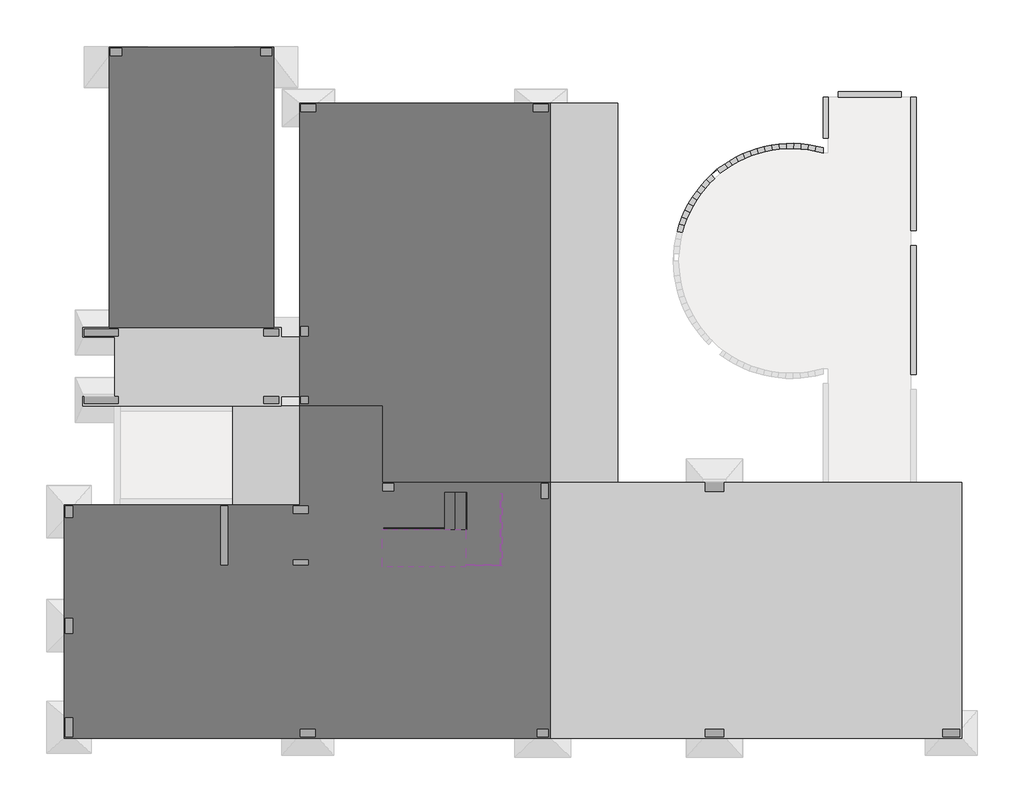
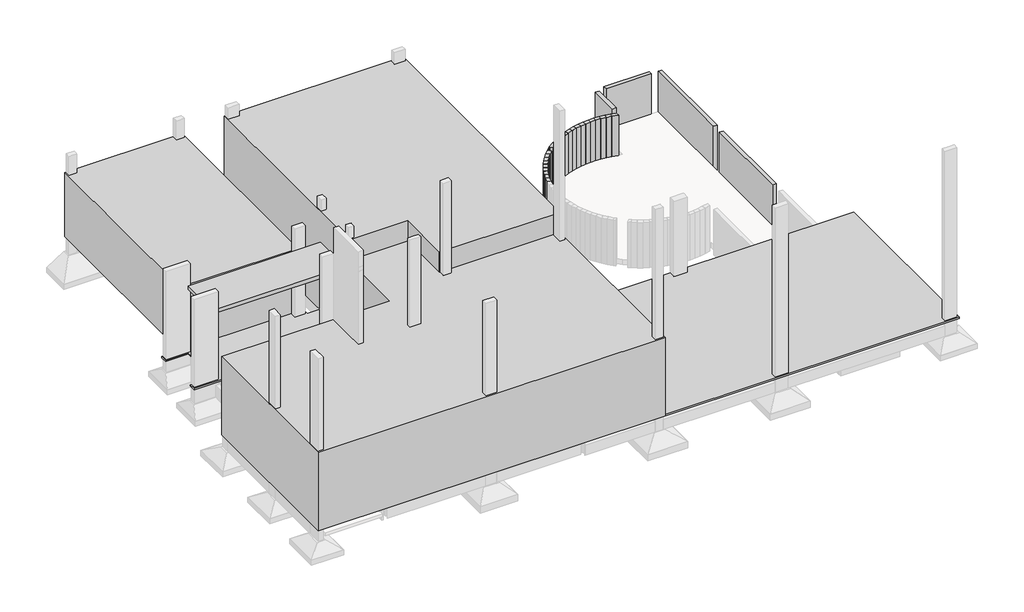
# One storey, part 4 of 4: 27 beams, 7 proxies, 6 railings, 2 stair flights, 1 slab.
"""IFC4 building model written with IfcOpenShell, lengths in millimetres."""

import ifcopenshell
import ifcopenshell.guid

model = None  # the IFC model being written
_history = None  # IfcOwnerHistory: only IFC2X3 demands one
_inside = {}  # id of a spatial element -> (the spatial element, [elements in it])
_under = {}  # id of a project, library or spatial element -> (it, [spatial elements below it])
_declared = {}  # id of a project -> (the project, [libraries it declares])
_typed = {}  # id of a type object -> (the type object, [elements of that type])
_made_of = {}  # id of a material, layer set ... -> (it, [elements and type objects made of it])


def new_model(schema):
    """Start an empty IFC model of exactly this schema.

    Asked for "IFC4X3", IfcOpenShell would pick the latest addendum, in which some entities
    have other attributes; the version numbers below select the first issue.
    IFC2X3 requires an IfcOwnerHistory on every rooted entity: one is made here for all.
    """
    global model, _history
    if schema == "IFC4X3":
        model = ifcopenshell.file(schema_version=(4, 3, 0, 0))
    else:
        model = ifcopenshell.file(schema=schema)
    _inside.clear()
    _under.clear()
    _declared.clear()
    _typed.clear()
    _made_of.clear()
    _history = None
    if model.schema == "IFC2X3":
        org = make("IfcOrganization", Name="unknown")
        user = make(
            "IfcPersonAndOrganization",
            ThePerson=make("IfcPerson", FamilyName="unknown"),
            TheOrganization=org,
        )
        app = make(
            "IfcApplication",
            ApplicationDeveloper=org,
            Version="unknown",
            ApplicationFullName="unknown",
            ApplicationIdentifier="unknown",
        )
        _history = make(
            "IfcOwnerHistory",
            OwningUser=user,
            OwningApplication=app,
            ChangeAction="ADDED",
            CreationDate=0,
        )
    return model


def make(cls, **values):
    """One entity of the class cls with the attributes given. An attribute that is None is left unset."""
    return model.create_entity(
        cls, **{name: value for name, value in values.items() if value is not None}
    )


def rooted(cls, **values):
    """An entity with a GlobalId (a new one), such as an element, a storey or a relation."""
    return make(cls, GlobalId=ifcopenshell.guid.new(), OwnerHistory=_history, **values)


def si_unit(unit_type, name, prefix=None):
    """IfcSIUnit, for example si_unit("LENGTHUNIT", "METRE", prefix="MILLI")."""
    return make("IfcSIUnit", UnitType=unit_type, Prefix=prefix, Name=name)


def assignment(units):
    """IfcUnitAssignment: the units of a project."""
    return None if units is None else make("IfcUnitAssignment", Units=units)


def point(xyz):
    """IfcCartesianPoint."""
    return None if xyz is None else make("IfcCartesianPoint", Coordinates=xyz)


def direction(xyz):
    """IfcDirection."""
    return None if xyz is None else make("IfcDirection", DirectionRatios=xyz)


def frame(location, z_axis=None, x_axis=None):
    """IfcAxis2Placement3D, a coordinate frame: its origin and axes. An axis left out is left unset."""
    return make(
        "IfcAxis2Placement3D",
        Location=point(location),
        Axis=direction(z_axis),
        RefDirection=direction(x_axis),
    )


def origin():
    """The frame at (0, 0, 0) with its axes left unset."""
    return frame((0.0, 0.0, 0.0))


def place(relative_to, where):
    """IfcLocalPlacement: puts the frame where relative to a parent placement (None: the world)."""
    return make(
        "IfcLocalPlacement", PlacementRelTo=relative_to, RelativePlacement=where
    )


def context(
    kind, dimensions, precision=None, world=None, true_north=None, identifier=None
):
    """IfcGeometricRepresentationContext, for example the 3D "Model" context."""
    return make(
        "IfcGeometricRepresentationContext",
        ContextIdentifier=identifier,
        ContextType=kind,
        CoordinateSpaceDimension=dimensions,
        Precision=precision,
        WorldCoordinateSystem=world,
        TrueNorth=true_north,
    )


def project(units=None, contexts=None):
    """IfcProject with its units and contexts."""
    return rooted(
        "IfcProject",
        Name="project",
        RepresentationContexts=contexts,
        UnitsInContext=assignment(units),
    )


def spatial(cls, under=None, at=None, **own):
    """A site, building, storey or space (cls), placed at a placement, below another one or the project."""
    s = rooted(cls, ObjectPlacement=at, **own)
    if under is not None:
        _under.setdefault(under.id(), (under, []))[1].append(s)
    return s


def polyline(points):
    """IfcPolyline through the points."""
    return make("IfcPolyline", Points=[point(p) for p in points])


def outline(outer, holes=None, kind="AREA"):
    """IfcArbitraryClosedProfileDef: a profile drawn as a closed curve; with holes, ...WithVoids."""
    if holes is None:
        return make("IfcArbitraryClosedProfileDef", ProfileType=kind, OuterCurve=outer)
    return make(
        "IfcArbitraryProfileDefWithVoids",
        ProfileType=kind,
        OuterCurve=outer,
        InnerCurves=holes,
    )


def extrude(swept, where, along, depth):
    """IfcExtrudedAreaSolid: the profile swept, set in the frame where, extruded along a direction by depth."""
    return make(
        "IfcExtrudedAreaSolid",
        SweptArea=swept,
        Position=where,
        ExtrudedDirection=direction(along),
        Depth=depth,
    )


def faces_of(points, faces, orient=None, outer=None):
    """IfcFace entities. A face is a list of loops; a loop is a list of indices into points, from 0.

    orient and outer hold one flag for each loop. By default every Orientation is true, the
    first loop of a face is its IfcFaceOuterBound and the others are IfcFaceBound.
    """
    made = []
    for i, loops in enumerate(faces):
        bounds = []
        for j, loop in enumerate(loops):
            is_outer = j == 0 if outer is None else outer[i][j]
            bounds.append(
                make(
                    "IfcFaceOuterBound" if is_outer else "IfcFaceBound",
                    Bound=make("IfcPolyLoop", Polygon=[points[k] for k in loop]),
                    Orientation=True if orient is None else orient[i][j],
                )
            )
        made.append(make("IfcFace", Bounds=bounds))
    return made


def faceted_brep(points, faces, orient=None, outer=None, voids=None):
    """IfcFacetedBrep: a solid bounded by flat faces; with voids (closed shells), ...WithVoids."""
    shared = [point(p) for p in points]
    hull = make("IfcClosedShell", CfsFaces=faces_of(shared, faces, orient, outer))
    if voids is None:
        return make("IfcFacetedBrep", Outer=hull)
    return make(
        "IfcFacetedBrepWithVoids",
        Outer=hull,
        Voids=[
            make(cls, CfsFaces=faces_of(shared, fs, o, b)) for cls, fs, o, b in voids
        ],
    )


def shape(context_of_items, identifier, shape_type, items):
    """IfcShapeRepresentation: the items that make up one representation, for example the "Body"."""
    return make(
        "IfcShapeRepresentation",
        ContextOfItems=context_of_items,
        RepresentationIdentifier=identifier,
        RepresentationType=shape_type,
        Items=items,
    )


def source(mapping_origin, context_of_items, identifier, shape_type, items):
    """IfcRepresentationMap: a shape defined once, which mapped items show again and again."""
    return make(
        "IfcRepresentationMap",
        MappingOrigin=mapping_origin,
        MappedRepresentation=shape(context_of_items, identifier, shape_type, items),
    )


def transform(
    local_origin,
    x_axis=None,
    y_axis=None,
    z_axis=None,
    scale=None,
    scale2=None,
    scale3=None,
    uniform=True,
):
    """IfcCartesianTransformationOperator3D, or its non-uniform kind. x_axis, y_axis, z_axis: its Axis1, 2, 3."""
    if uniform:
        return make(
            "IfcCartesianTransformationOperator3D",
            Axis1=direction(x_axis),
            Axis2=direction(y_axis),
            LocalOrigin=point(local_origin),
            Scale=scale,
            Axis3=direction(z_axis),
        )
    return make(
        "IfcCartesianTransformationOperator3DnonUniform",
        Axis1=direction(x_axis),
        Axis2=direction(y_axis),
        LocalOrigin=point(local_origin),
        Scale=scale,
        Axis3=direction(z_axis),
        Scale2=scale2,
        Scale3=scale3,
    )


def mapped(mapping_source, mapping_target):
    """IfcMappedItem: shows the shape of a source again, moved by a transform."""
    return make(
        "IfcMappedItem", MappingSource=mapping_source, MappingTarget=mapping_target
    )


def made_of(thing, what):
    """Note that an element or type object is made of a material, layer set ...; save() writes the relation."""
    if what is not None:
        _made_of.setdefault(what.id(), (what, []))[1].append(thing)
    return thing


def element(
    cls,
    number,
    at=None,
    inside=None,
    cuts=None,
    type_object=None,
    material=None,
    context=None,
    identifier="Body",
    shape_type=None,
    held_by="IfcProductDefinitionShape",
    body=None,
    shapes=None,
    **own,
):
    """One element of the class cls, such as IfcWall. Its Tag is "e" and its number.

    at: its placement. inside: the storey or other place that contains it. cuts: it is an
    opening in that element (IfcRelVoidsElement). A single representation is given by context,
    identifier, shape_type and body (its items); several are given by shapes. held_by: the class
    of the entity that holds the representations. save() writes the other relations.
    """
    e = rooted(cls, Tag="e%d" % number, ObjectPlacement=at, **own)
    if body is not None:
        shapes = [shape(context, identifier, shape_type, body)]
    if shapes is not None:
        e.Representation = make(held_by, Representations=shapes)
    if inside is not None:
        _inside.setdefault(inside.id(), (inside, []))[1].append(e)
    if cuts is not None:
        rooted(
            "IfcRelVoidsElement", RelatingBuildingElement=cuts, RelatedOpeningElement=e
        )
    if type_object is not None:
        _typed.setdefault(type_object.id(), (type_object, []))[1].append(e)
    return made_of(e, material)


def aggregate(whole, parts):
    """IfcRelAggregates: a whole, such as a stair, and the parts it consists of."""
    return rooted("IfcRelAggregates", RelatingObject=whole, RelatedObjects=parts)


def save(model, path):
    """Write the relations noted so far, then the file.

    IfcRelAggregates (storeys below a building ...), IfcRelContainedInSpatialStructure (elements
    in a storey), IfcRelDefinesByType, IfcRelAssociatesMaterial and IfcRelDeclares: one each for
    every whole, place, type object, material and project.
    """
    for whole, parts in _under.values():
        aggregate(whole, parts)
    for where, things in _inside.values():
        rooted(
            "IfcRelContainedInSpatialStructure",
            RelatedElements=things,
            RelatingStructure=where,
        )
    for kind, things in _typed.values():
        rooted("IfcRelDefinesByType", RelatedObjects=things, RelatingType=kind)
    for what, things in _made_of.values():
        rooted("IfcRelAssociatesMaterial", RelatedObjects=things, RelatingMaterial=what)
    for by, libraries in _declared.values():
        rooted("IfcRelDeclares", RelatingContext=by, RelatedDefinitions=libraries)
    model.write(path)


def railing_81dbcb3b(model_context):
    return source(origin(), model_context, "Body", "SweptSolid", [
        extrude(outline(polyline([(1832.4523952, 3702.0), (1832.4523952, 3594.0), (1856.4523952, 3594.0), (1856.4523952, 3702.0), (1866.9523952, 3702.0), (1866.9523952, 3700.0), (1858.4523952, 3700.0), (1858.4523952, 3592.0), (1830.4523952, 3592.0), (1830.4523952, 3700.0), (1821.9523952, 3700.0), (1821.9523952, 3702.0), (1832.4523952, 3702.0)])), frame((-12226.1487231, 0.0, 0.0), z_axis=(1.0, 0.0, 0.0), x_axis=(0.0, 1.0, 0.0)), (0.0, 0.0, 1.0), 1940.0),
    ])


def railing_0d959ca4(model_context):
    return source(origin(), model_context, "Body", "SweptSolid", [
        extrude(outline(polyline([(-4674.5702584, 2133.3602771), (-4674.5702584, 2121.3602771), (-6610.5702584, 2121.3602771), (-6610.5702584, 2133.3602771), (-4674.5702584, 2133.3602771)])), frame((0.0, 0.0, 4122.0679199), z_axis=(0.0, 0.0, 1.0), x_axis=(1.0, 0.0, 0.0)), (0.0, 0.0, 1.0), 1100.0),
    ])


def railing_24874f95(model_context):
    return source(origin(), model_context, "Body", "SweptSolid", [
        extrude(outline(polyline([(1832.4523952, 3702.0), (1832.4523952, 3594.0), (1856.4523952, 3594.0), (1856.4523952, 3702.0), (1866.9523952, 3702.0), (1866.9523952, 3700.0), (1858.4523952, 3700.0), (1858.4523952, 3592.0), (1830.4523952, 3592.0), (1830.4523952, 3700.0), (1821.9523952, 3700.0), (1821.9523952, 3702.0), (1832.4523952, 3702.0)])), frame((-12226.1487231, 0.0, 0.0), z_axis=(1.0, 0.0, 0.0), x_axis=(0.0, 1.0, 0.0)), (0.0, 0.0, 1.0), 925.0),
    ])


def railing_29f9e2f6(model_context):
    return source(origin(), model_context, "Body", "SweptSolid", [
        extrude(outline(polyline([(-4674.5702584, 2133.3602771), (-4674.5702584, 2121.3602771), (-5595.5702584, 2121.3602771), (-5595.5702584, 2133.3602771), (-4674.5702584, 2133.3602771)])), frame((0.0, 0.0, 4122.0679199), z_axis=(0.0, 0.0, 1.0), x_axis=(1.0, 0.0, 0.0)), (0.0, 0.0, 1.0), 1100.0),
    ])


def railing_c44cfcee(model_context):
    return source(origin(), model_context, "Body", "SweptSolid", [
        extrude(outline(polyline([(1672.2222222, -4460.281307), (500.0, -4460.281307), (1877.7777778, -2220.281307), (3050.0, -2220.281307), (1672.2222222, -4460.281307)])), frame((0.0, -5573.3699847, 0.0), z_axis=(0.0, 1.0, 0.0), x_axis=(0.0, 0.0, 1.0)), (0.0, 0.0, 1.0), 12.0),
    ])


model = new_model("IFC4")

# Units and contexts
model_context = context("Model", 3, world=origin())
ifc_project = project(units=[si_unit("LENGTHUNIT", "METRE", prefix="MILLI")], contexts=[model_context])

# Site, building, storey
site = spatial("IfcSite", under=ifc_project)
building = spatial("IfcBuilding", under=site)
storey = spatial("IfcBuildingStorey", under=building, Name="PAVIMENTO TÉRREO", Elevation=500.0)

# Beams
placement = place(None, origin())
element("IfcBeam", 1, ObjectType="TQS - Viga retangular : 14.0 x 180.0", at=placement, inside=storey, context=model_context, shape_type="SweptSolid", body=[
    extrude(outline(polyline([(9422.718693, 6109.4300153), (9422.718693, 5969.4300153), (7734.718693, 5969.4300153), (7734.718693, 6109.4300153), (9422.718693, 6109.4300153)])), frame((0.0, 0.0, -1450.0), z_axis=(0.0, 0.0, 1.0), x_axis=(1.0, 0.0, 0.0)), (0.0, 0.0, 1.0), 1800.0),
])
element("IfcBeam", 2, ObjectType="TQS - Viga retangular : 14.0 x 180.0", at=placement, inside=storey, context=model_context, shape_type="Brep", body=[
    faceted_brep([(3491.8466557, 2568.9190116, 350.0), (3435.4949989, 2377.433408, 350.0), (3571.057344, 2342.1816685, 350.0), (3624.8943566, 2525.1223914, 350.0), (3571.057344, 2342.1816685, -1250.0), (3571.057344, 2342.1816685, -1450.0), (3624.8943566, 2525.1223914, -1450.0), (3624.8943566, 2525.1223914, -1250.0), (3435.4949989, 2377.433408, -1450.0), (3491.8466557, 2568.9190116, -1450.0)], [[[0, 1, 2, 3]], [[3, 2, 4, 5, 6, 7]], [[6, 5, 8, 9]], [[1, 0, 9, 8]], [[1, 8, 5, 4, 2]], [[0, 3, 7, 6, 9]]]),
])
element("IfcBeam", 3, ObjectType="TQS - Viga retangular : 14.0 x 180.0", at=placement, inside=storey, context=model_context, shape_type="Brep", body=[
    faceted_brep([(3560.4750252, 2757.0390761, 350.0), (3491.8466557, 2568.9190116, 350.0), (3624.8943566, 2525.1223914, 350.0), (3690.4700641, 2704.8746778, 350.0), (3624.8943566, 2525.1223914, -1250.0), (3624.8943566, 2525.1223914, -1450.0), (3690.4700641, 2704.8746778, -1450.0), (3690.4700641, 2704.8746778, -1250.0), (3491.8466557, 2568.9190116, -1450.0), (3560.4750252, 2757.0390761, -1450.0)], [[[0, 1, 2, 3]], [[3, 2, 4, 5, 6, 7]], [[6, 5, 8, 9]], [[1, 0, 9, 8]], [[1, 8, 5, 4, 2]], [[0, 3, 7, 6, 9]]]),
])
element("IfcBeam", 4, ObjectType="TQS - Viga retangular : 14.0 x 180.0", at=placement, inside=storey, context=model_context, shape_type="Brep", body=[
    faceted_brep([(3640.6668309, 2939.8368394, 350.0), (3560.4750252, 2757.0390761, 350.0), (3690.4700641, 2704.8746778, 350.0), (3767.0835383, 2879.5156103, 350.0), (3690.4700641, 2704.8746778, -1250.0), (3690.4700641, 2704.8746778, -1450.0), (3767.0835383, 2879.5156103, -1450.0), (3767.0835383, 2879.5156103, -1250.0), (3560.4750252, 2757.0390761, -1450.0), (3640.6668309, 2939.8368394, -1450.0)], [[[0, 1, 2, 3]], [[3, 2, 4, 5, 6, 7]], [[6, 5, 8, 9]], [[1, 0, 9, 8]], [[1, 8, 5, 4, 2]], [[0, 3, 7, 6, 9]]]),
])
element("IfcBeam", 5, ObjectType="TQS - Viga retangular : 14.0 x 180.0", at=placement, inside=storey, context=model_context, shape_type="Brep", body=[
    faceted_brep([(3732.4184841, 3117.3686176, 350.0), (3640.6668309, 2939.8368394, 350.0), (3767.0835383, 2879.5156103, 350.0), (3854.7456543, 3049.1344759, 350.0), (3767.0835383, 2879.5156103, -1250.0), (3767.0835383, 2879.5156103, -1450.0), (3854.7456543, 3049.1344759, -1450.0), (3854.7456543, 3049.1344759, -1250.0), (3640.6668309, 2939.8368394, -1450.0), (3732.4184841, 3117.3686176, -1450.0)], [[[0, 1, 2, 3]], [[3, 2, 4, 5, 6, 7]], [[6, 5, 8, 9]], [[1, 0, 9, 8]], [[1, 8, 5, 4, 2]], [[0, 3, 7, 6, 9]]]),
])
element("IfcBeam", 6, ObjectType="TQS - Viga retangular : 14.0 x 180.0", at=placement, inside=storey, context=model_context, shape_type="Brep", body=[
    faceted_brep([(3835.4781404, 3289.0593829, 350.0), (3732.4184841, 3117.3686176, 350.0), (3854.7456543, 3049.1344759, 350.0), (3953.2211063, 3213.1882515, 350.0), (3854.7456543, 3049.1344759, -1250.0), (3854.7456543, 3049.1344759, -1450.0), (3953.2211063, 3213.1882515, -1450.0), (3953.2211063, 3213.1882515, -1250.0), (3732.4184841, 3117.3686176, -1450.0), (3835.4781404, 3289.0593829, -1450.0)], [[[0, 1, 2, 3]], [[3, 2, 4, 5, 6, 7]], [[6, 5, 8, 9]], [[1, 0, 9, 8]], [[1, 8, 5, 4, 2]], [[0, 3, 7, 6, 9]]]),
])
element("IfcBeam", 7, ObjectType="TQS - Viga retangular : 14.0 x 180.0", at=placement, inside=storey, context=model_context, shape_type="Brep", body=[
    faceted_brep([(3949.2418511, 3453.852677, 350.0), (3835.4781404, 3289.0593829, 350.0), (3953.2211063, 3213.1882515, 350.0), (4061.9244879, 3370.6513671, 350.0), (3953.2211063, 3213.1882515, -1250.0), (3953.2211063, 3213.1882515, -1450.0), (4061.9244879, 3370.6513671, -1450.0), (4061.9244879, 3370.6513671, -1250.0), (3835.4781404, 3289.0593829, -1450.0), (3949.2418511, 3453.852677, -1450.0)], [[[0, 1, 2, 3]], [[3, 2, 4, 5, 6, 7]], [[6, 5, 8, 9]], [[1, 0, 9, 8]], [[1, 8, 5, 4, 2]], [[0, 3, 7, 6, 9]]]),
])
element("IfcBeam", 8, ObjectType="TQS - Viga retangular : 14.0 x 180.0", at=placement, inside=storey, context=model_context, shape_type="Brep", body=[
    faceted_brep([(4073.2495799, 3611.0821108, 350.0), (3949.2418511, 3453.852677, 350.0), (4061.9244879, 3370.6513671, 350.0), (4180.416223, 3520.8870709, 350.0), (4061.9244879, 3370.6513671, -1250.0), (4061.9244879, 3370.6513671, -1450.0), (4180.416223, 3520.8870709, -1450.0), (4180.416223, 3520.8870709, -1250.0), (3949.2418511, 3453.852677, -1450.0), (4073.2495799, 3611.0821108, -1450.0)], [[[0, 1, 2, 3]], [[3, 2, 4, 5, 6, 7]], [[6, 5, 8, 9]], [[1, 0, 9, 8]], [[1, 8, 5, 4, 2]], [[0, 3, 7, 6, 9]]]),
])
element("IfcBeam", 9, ObjectType="TQS - Viga retangular : 14.0 x 180.0", at=placement, inside=storey, context=model_context, shape_type="Brep", body=[
    faceted_brep([(4206.9998658, 3760.1118816, 350.0), (4073.2495799, 3611.0821108, 350.0), (4180.416223, 3520.8870709, 350.0), (4308.2171619, 3663.2878479, 350.0), (4180.416223, 3520.8870709, -1250.0), (4180.416223, 3520.8870709, -1450.0), (4308.2171619, 3663.2878479, -1450.0), (4308.2171619, 3663.2878479, -1250.0), (4073.2495799, 3611.0821108, -1450.0), (4206.9998658, 3760.1118816, -1450.0)], [[[0, 1, 2, 3]], [[3, 2, 4, 5, 6, 7]], [[6, 5, 8, 9]], [[1, 0, 9, 8]], [[1, 8, 5, 4, 2]], [[0, 3, 7, 6, 9]]]),
])
element("IfcBeam", 10, ObjectType="TQS - Viga retangular : 14.0 x 180.0", at=placement, inside=storey, context=model_context, shape_type="Brep", body=[
    faceted_brep([(4505.0858129, 4030.990239, 350.0), (4495.3853819, 4043.0011294, 350.0), (4357.8172159, 3908.0548411, 350.0), (4500.8039544, 4027.7001668, 350.0), (4495.3853819, 4043.0011294, -1450.0), (4505.0858129, 4030.990239, -1450.0), (4500.8039544, 4027.7001668, -1450.0), (4357.8172159, 3908.0548411, -1450.0)], [[[0, 1, 2, 3]], [[4, 5, 6, 7]], [[1, 4, 7, 2]], [[4, 1, 0, 5]], [[3, 6, 5, 0]], [[6, 3, 2, 7]]]),
    faceted_brep([(4433.7325967, 3786.411115, 350.0), (4308.2171619, 3663.2878479, 350.0), (4308.2171619, 3663.2878479, -1250.0), (4308.2171619, 3663.2878479, -1450.0), (4433.7325967, 3786.411115, -1450.0), (4433.7325967, 3786.411115, -1250.0), (4346.9865149, 3897.4305598, 350.0), (4346.9865149, 3897.4305598, -1450.0), (4206.9998658, 3760.1118816, 350.0), (4206.9998658, 3760.1118816, -1450.0)], [[[0, 1, 2, 3, 4, 5]], [[6, 0, 5, 4, 7]], [[8, 9, 3, 2, 1]], [[1, 0, 6, 8]], [[4, 3, 9, 7]], [[6, 7, 9, 8]]]),
])
element("IfcBeam", 11, ObjectType="TQS - Viga retangular : 14.0 x 180.0", at=placement, inside=storey, context=model_context, shape_type="Brep", body=[
    faceted_brep([(4707.2476524, 4182.7114576, 350.0), (4495.3853819, 4043.0011294, 350.0), (4505.0858129, 4030.990239, 350.0), (4583.7591724, 3933.5783713, 350.0), (4784.4362281, 4065.9127281, 350.0), (4583.7591724, 3933.5783713, -1450.0), (4742.6545701, 4038.3602567, -1450.0), (4784.4362281, 4065.9127281, -1450.0), (4784.4362281, 4065.9127281, -1250.0), (4495.3853819, 4043.0011294, -1450.0), (4707.2476524, 4182.7114576, -1450.0), (4505.0858129, 4030.990239, -1450.0)], [[[0, 1, 2, 3, 4]], [[4, 3, 5, 6, 7, 8]], [[9, 10, 7, 6, 5, 11]], [[1, 0, 10, 9]], [[1, 9, 11, 5, 3, 2]], [[0, 4, 8, 7, 10]]]),
])
element("IfcBeam", 12, ObjectType="TQS - Viga retangular : 14.0 x 180.0", at=placement, inside=storey, context=model_context, shape_type="Brep", body=[
    faceted_brep([(4828.0654459, 4262.728967, 350.0), (4707.2476524, 4182.7114576, 350.0), (4784.4362281, 4065.9127281, 350.0), (4901.6570883, 4143.547992, 350.0), (4784.4362281, 4065.9127281, -1250.0), (4784.4362281, 4065.9127281, -1450.0), (4901.6570883, 4143.547992, -1450.0), (4901.6570883, 4143.547992, -1250.0), (4707.2476524, 4182.7114576, -1450.0), (4828.0654459, 4262.728967, -1450.0)], [[[0, 1, 2, 3]], [[3, 2, 4, 5, 6, 7]], [[6, 5, 8, 9]], [[1, 0, 9, 8]], [[1, 8, 5, 4, 2]], [[0, 3, 7, 6, 9]]]),
])
element("IfcBeam", 13, ObjectType="TQS - Viga retangular : 14.0 x 180.0", at=placement, inside=storey, context=model_context, shape_type="Brep", body=[
    faceted_brep([(5001.7073563, 4362.4661134, 350.0), (4828.0654459, 4262.728967, 350.0), (4901.6570883, 4143.547992, 350.0), (5067.5752245, 4238.8487257, 350.0), (4901.6570883, 4143.547992, -1250.0), (4901.6570883, 4143.547992, -1450.0), (5067.5752245, 4238.8487257, -1450.0), (5067.5752245, 4238.8487257, -1250.0), (4828.0654459, 4262.728967, -1450.0), (5001.7073563, 4362.4661134, -1450.0)], [[[0, 1, 2, 3]], [[3, 2, 4, 5, 6, 7]], [[6, 5, 8, 9]], [[1, 0, 9, 8]], [[1, 8, 5, 4, 2]], [[0, 3, 7, 6, 9]]]),
])
element("IfcBeam", 14, ObjectType="TQS - Viga retangular : 14.0 x 180.0", at=placement, inside=storey, context=model_context, shape_type="Brep", body=[
    faceted_brep([(5181.3373377, 4450.9651597, 350.0), (5001.7073563, 4362.4661134, 350.0), (5067.5752245, 4238.8487257, 350.0), (5239.2150761, 4323.4112417, 350.0), (5067.5752245, 4238.8487257, -1250.0), (5067.5752245, 4238.8487257, -1450.0), (5239.2150761, 4323.4112417, -1450.0), (5239.2150761, 4323.4112417, -1250.0), (5001.7073563, 4362.4661134, -1450.0), (5181.3373377, 4450.9651597, -1450.0)], [[[0, 1, 2, 3]], [[3, 2, 4, 5, 6, 7]], [[6, 5, 8, 9]], [[1, 0, 9, 8]], [[1, 8, 5, 4, 2]], [[0, 3, 7, 6, 9]]]),
])
element("IfcBeam", 15, ObjectType="TQS - Viga retangular : 14.0 x 180.0", at=placement, inside=storey, context=model_context, shape_type="Brep", body=[
    faceted_brep([(5366.2290044, 4527.8682345, 350.0), (5181.3373377, 4450.9651597, 350.0), (5239.2150761, 4323.4112417, 350.0), (5415.8825678, 4396.8935871, 350.0), (5239.2150761, 4323.4112417, -1250.0), (5239.2150761, 4323.4112417, -1450.0), (5415.8825678, 4396.8935871, -1450.0), (5415.8825678, 4396.8935871, -1250.0), (5181.3373377, 4450.9651597, -1450.0), (5366.2290044, 4527.8682345, -1450.0)], [[[0, 1, 2, 3]], [[3, 2, 4, 5, 6, 7]], [[6, 5, 8, 9]], [[1, 0, 9, 8]], [[1, 8, 5, 4, 2]], [[0, 3, 7, 6, 9]]]),
])
element("IfcBeam", 16, ObjectType="TQS - Viga retangular : 14.0 x 180.0", at=placement, inside=storey, context=model_context, shape_type="Brep", body=[
    faceted_brep([(5555.634694, 4592.8643582, 350.0), (5366.2290044, 4527.8682345, 350.0), (5415.8825678, 4396.8935871, 350.0), (5596.8632938, 4458.9986151, 350.0), (5415.8825678, 4396.8935871, -1250.0), (5415.8825678, 4396.8935871, -1450.0), (5596.8632938, 4458.9986151, -1450.0), (5596.8632938, 4458.9986151, -1250.0), (5366.2290044, 4527.8682345, -1450.0), (5555.634694, 4592.8643582, -1450.0)], [[[0, 1, 2, 3]], [[3, 2, 4, 5, 6, 7]], [[6, 5, 8, 9]], [[1, 0, 9, 8]], [[1, 8, 5, 4, 2]], [[0, 3, 7, 6, 9]]]),
])
element("IfcBeam", 17, ObjectType="TQS - Viga retangular : 14.0 x 180.0", at=placement, inside=storey, context=model_context, shape_type="Brep", body=[
    faceted_brep([(5748.78849, 4645.6907002, 350.0), (5555.634694, 4592.8643582, 350.0), (5596.8632938, 4458.9986151, 350.0), (5781.4254065, 4509.475186, 350.0), (5596.8632938, 4458.9986151, -1250.0), (5596.8632938, 4458.9986151, -1450.0), (5781.4254065, 4509.475186, -1450.0), (5781.4254065, 4509.475186, -1250.0), (5555.634694, 4592.8643582, -1450.0), (5748.78849, 4645.6907002, -1450.0)], [[[0, 1, 2, 3]], [[3, 2, 4, 5, 6, 7]], [[6, 5, 8, 9]], [[1, 0, 9, 8]], [[1, 8, 5, 4, 2]], [[0, 3, 7, 6, 9]]]),
])
element("IfcBeam", 18, ObjectType="TQS - Viga retangular : 14.0 x 180.0", at=placement, inside=storey, context=model_context, shape_type="Brep", body=[
    faceted_brep([(5944.9093194, 4686.133642, 350.0), (5748.78849, 4645.6907002, 350.0), (5781.4254065, 4509.475186, 350.0), (5968.8225759, 4548.1191834, 350.0), (5781.4254065, 4509.475186, -1250.0), (5781.4254065, 4509.475186, -1450.0), (5968.8225759, 4548.1191834, -1450.0), (5968.8225759, 4548.1191834, -1250.0), (5748.78849, 4645.6907002, -1450.0), (5944.9093194, 4686.133642, -1450.0)], [[[0, 1, 2, 3]], [[3, 2, 4, 5, 6, 7]], [[6, 5, 8, 9]], [[1, 0, 9, 8]], [[1, 8, 5, 4, 2]], [[0, 3, 7, 6, 9]]]),
])
element("IfcBeam", 19, ObjectType="TQS - Viga retangular : 14.0 x 180.0", at=placement, inside=storey, context=model_context, shape_type="Brep", body=[
    faceted_brep([(6143.2041112, 4714.029641, 350.0), (5944.9093194, 4686.133642, 350.0), (5968.8225759, 4548.1191834, 350.0), (6158.2970076, 4574.7743392, 350.0), (5968.8225759, 4548.1191834, -1250.0), (5968.8225759, 4548.1191834, -1450.0), (6158.2970076, 4574.7743392, -1450.0), (6158.2970076, 4574.7743392, -1250.0), (5944.9093194, 4686.133642, -1450.0), (6143.2041112, 4714.029641, -1450.0)], [[[0, 1, 2, 3]], [[3, 2, 4, 5, 6, 7]], [[6, 5, 8, 9]], [[1, 0, 9, 8]], [[1, 8, 5, 4, 2]], [[0, 3, 7, 6, 9]]]),
])
element("IfcBeam", 20, ObjectType="TQS - Viga retangular : 14.0 x 180.0", at=placement, inside=storey, context=model_context, shape_type="Brep", body=[
    faceted_brep([(6342.8710035, 4729.2658917, 350.0), (6143.2041112, 4714.029641, 350.0), (6158.2970076, 4574.7743392, 350.0), (6349.0825072, 4589.3328655, 350.0), (6158.2970076, 4574.7743392, -1250.0), (6158.2970076, 4574.7743392, -1450.0), (6349.0825072, 4589.3328655, -1450.0), (6349.0825072, 4589.3328655, -1250.0), (6143.2041112, 4714.029641, -1450.0), (6342.8710035, 4729.2658917, -1450.0)], [[[0, 1, 2, 3]], [[3, 2, 4, 5, 6, 7]], [[6, 5, 8, 9]], [[1, 0, 9, 8]], [[1, 8, 5, 4, 2]], [[0, 3, 7, 6, 9]]]),
])
element("IfcBeam", 21, ObjectType="TQS - Viga retangular : 14.0 x 180.0", at=placement, inside=storey, context=model_context, shape_type="Brep", body=[
    faceted_brep([(6543.1025857, 4731.7807819, 350.0), (6342.8710035, 4729.2658917, 350.0), (6349.0825072, 4589.3328655, 350.0), (6540.4075788, 4591.7358908, 350.0), (6349.0825072, 4589.3328655, -1250.0), (6349.0825072, 4589.3328655, -1450.0), (6540.4075788, 4591.7358908, -1450.0), (6540.4075788, 4591.7358908, -1250.0), (6342.8710035, 4729.2658917, -1450.0), (6543.1025857, 4731.7807819, -1450.0)], [[[0, 1, 2, 3]], [[3, 2, 4, 5, 6, 7]], [[6, 5, 8, 9]], [[1, 0, 9, 8]], [[1, 8, 5, 4, 2]], [[0, 3, 7, 6, 9]]]),
])
element("IfcBeam", 22, ObjectType="TQS - Viga retangular : 14.0 x 180.0", at=placement, inside=storey, context=model_context, shape_type="Brep", body=[
    faceted_brep([(6743.0891637, 4721.5641421, 350.0), (6543.1025857, 4731.7807819, 350.0), (6540.4075788, 4591.7358908, 350.0), (6731.4985443, 4581.9736977, 350.0), (6540.4075788, 4591.7358908, -1250.0), (6540.4075788, 4591.7358908, -1450.0), (6731.4985443, 4581.9736977, -1450.0), (6731.4985443, 4581.9736977, -1250.0), (6543.1025857, 4731.7807819, -1450.0), (6743.0891637, 4721.5641421, -1450.0)], [[[0, 1, 2, 3]], [[3, 2, 4, 5, 6, 7]], [[6, 5, 8, 9]], [[1, 0, 9, 8]], [[1, 8, 5, 4, 2]], [[0, 3, 7, 6, 9]]]),
])
element("IfcBeam", 23, ObjectType="TQS - Viga retangular : 14.0 x 180.0", at=placement, inside=storey, context=model_context, shape_type="Brep", body=[
    faceted_brep([(6942.0220345, 4698.657286, 350.0), (6743.0891637, 4721.5641421, 350.0), (6731.4985443, 4581.9736977, 350.0), (6921.5826725, 4560.0857626, 350.0), (6731.4985443, 4581.9736977, -1250.0), (6731.4985443, 4581.9736977, -1450.0), (6921.5826725, 4560.0857626, -1450.0), (6921.5826725, 4560.0857626, -1250.0), (6743.0891637, 4721.5641421, -1450.0), (6942.0220345, 4698.657286, -1450.0)], [[[0, 1, 2, 3]], [[3, 2, 4, 5, 6, 7]], [[6, 5, 8, 9]], [[1, 0, 9, 8]], [[1, 8, 5, 4, 2]], [[0, 3, 7, 6, 9]]]),
])
element("IfcBeam", 24, ObjectType="TQS - Viga retangular : 14.0 x 180.0", at=placement, inside=storey, context=model_context, shape_type="Brep", body=[
    faceted_brep([(7139.0967556, 4663.1528442, 350.0), (6942.0220345, 4698.657286, 350.0), (6921.5826725, 4560.0857626, 350.0), (7109.8912551, 4526.1606043, 350.0), (6921.5826725, 4560.0857626, -1250.0), (6921.5826725, 4560.0857626, -1450.0), (7109.8912551, 4526.1606043, -1450.0), (7109.8912551, 4526.1606043, -1250.0), (6942.0220345, 4698.657286, -1450.0), (7139.0967556, 4663.1528442, -1450.0)], [[[0, 1, 2, 3]], [[3, 2, 4, 5, 6, 7]], [[6, 5, 8, 9]], [[1, 0, 9, 8]], [[1, 8, 5, 4, 2]], [[0, 3, 7, 6, 9]]]),
])
element("IfcBeam", 25, ObjectType="TQS - Viga retangular : 14.0 x 180.0", at=placement, inside=storey, context=model_context, shape_type="Brep", body=[
    faceted_brep([(7109.8912551, 4526.1606043, 350.0), (7334.7218272, 4470.7003679, 350.0), (7334.7218272, 4614.8968948, 350.0), (7139.0967556, 4663.1528442, 350.0), (7109.8912551, 4526.1606043, -1250.0), (7109.8912551, 4526.1606043, -1450.0), (7334.7218272, 4470.7003679, -1450.0), (7334.7218272, 4470.7003679, -1250.0), (7139.0967556, 4663.1528442, -1450.0), (7334.7218272, 4614.8968948, -1450.0)], [[[0, 1, 2, 3]], [[1, 0, 4, 5, 6, 7]], [[6, 5, 8, 9]], [[3, 2, 9, 8]], [[2, 1, 7, 6, 9]], [[3, 8, 5, 4, 0]]]),
])
element("IfcBeam", 26, ObjectType="TQS - Viga retangular : 14.0 x 180.0", at=placement, inside=storey, context=model_context, shape_type="Brep", body=[
    faceted_brep([(7334.7218272, 5969.4300153, 350.0), (7334.7218272, 4870.7003679, 350.0), (7474.7218272, 4870.7003679, 350.0), (7474.7218272, 5969.4300153, 350.0), (7474.7218272, 4870.7003679, -1250.0), (7474.7218272, 4870.7003679, -1450.0), (7474.7218272, 5969.4300153, -1450.0), (7474.7218272, 5969.4300153, -1250.0), (7334.7218272, 4870.7003679, -1450.0), (7334.7218272, 5969.4300153, -1450.0)], [[[0, 1, 2, 3]], [[3, 2, 4, 5, 6, 7]], [[6, 5, 8, 9]], [[1, 0, 9, 8]], [[0, 3, 7, 6, 9]], [[1, 8, 5, 4, 2]]]),
])
element("IfcBeam", 27, ObjectType="TQS - Viga retangular : 14.0 x 180.0", at=placement, inside=storey, context=model_context, shape_type="Brep", body=[
    faceted_brep([(9822.718693, 5969.4300153, 350.0), (9682.718693, 5969.4300153, 350.0), (9682.718693, 2394.0144504, 350.0), (9822.718693, 2394.0144504, 350.0), (9822.718693, 5969.4300153, -1450.0), (9822.718693, 2394.0144504, -1450.0), (9682.718693, 5969.4300153, -1450.0), (9682.718693, 2394.0144504, -1450.0), (9682.718693, 5969.4300153, -1250.0)], [[[0, 1, 2, 3]], [[4, 0, 3, 5]], [[6, 4, 5, 7]], [[1, 8, 6, 7, 2]], [[3, 2, 7, 5]], [[1, 0, 4, 6, 8]]]),
    faceted_brep([(9822.718693, -1451.4011146, 350.0), (9682.718693, -1451.4011146, 350.0), (9682.718693, -1451.4011146, -1450.0), (9822.718693, -1451.4011146, -1450.0), (9682.718693, 1994.0144504, 350.0), (9822.718693, 1994.0144504, 350.0), (9822.718693, 1994.0144504, -1450.0), (9682.718693, 1994.0144504, -1450.0)], [[[0, 1, 2, 3]], [[4, 5, 6, 7]], [[1, 0, 5, 4]], [[0, 3, 6, 5]], [[3, 2, 7, 6]], [[2, 1, 4, 7]]]),
])

# Proxies
element("IfcBuildingElementProxy", 28, Name="GARAGEM : GARAGEM", ObjectType="GARAGEM : GARAGEM", at=placement, inside=storey, context=model_context, shape_type="SweptSolid", body=[
    extrude(outline(polyline([(-7360.281307, 7304.4300153), (-7360.281307, -195.5699847), (-11760.281307, -195.5699847), (-11760.281307, 7304.4300153), (-7360.281307, 7304.4300153)])), frame((0.0, 0.0, 500.0), z_axis=(0.0, 0.0, 1.0), x_axis=(1.0, 0.0, 0.0)), (0.0, 0.0, 1.0), 2550.0),
])
element("IfcBuildingElementProxy", 29, Name="PERGOLADO SALAS : PERGOLADO SALAS", ObjectType="PERGOLADO SALAS : PERGOLADO SALAS", at=placement, inside=storey, context=model_context, shape_type="SweptSolid", body=[
    extrude(outline(polyline([(1839.718693, 5804.4300153), (1839.718693, -4345.5699847), (39.718693, -4345.5699847), (39.718693, 5804.4300153), (1839.718693, 5804.4300153)])), frame((0.0, 0.0, 500.0), z_axis=(0.0, 0.0, 1.0), x_axis=(1.0, 0.0, 0.0)), (0.0, 0.0, 1.0), 50.0),
])
element("IfcBuildingElementProxy", 30, Name="VARANDA GOURMET : VARANDA GOURMET", ObjectType="VARANDA GOURMET : VARANDA GOURMET", at=placement, inside=storey, context=model_context, shape_type="SweptSolid", body=[
    extrude(outline(polyline([(11039.718693, -4345.5699847), (11039.718693, -11195.5699847), (39.718693, -11195.5699847), (39.718693, -4345.5699847), (11039.718693, -4345.5699847)])), frame((0.0, 0.0, 500.0), z_axis=(0.0, 0.0, 1.0), x_axis=(1.0, 0.0, 0.0)), (0.0, 0.0, 1.0), 50.0),
])
element("IfcBuildingElementProxy", 31, Name="PÓRTICO ENTRADA : PÓRTICO ENTRADA", ObjectType="PÓRTICO ENTRADA : PÓRTICO ENTRADA", at=placement, inside=storey, context=model_context, shape_type="SweptSolid", body=[
    extrude(outline(polyline([(-7160.281307, -445.5699847), (-6660.281307, -445.5699847), (-6660.281307, -2045.5699847), (-7160.281307, -2045.5699847), (-7160.281307, -2295.5699847), (-12460.281307, -2295.5699847), (-12460.281307, -2045.5699847), (-11610.281307, -2045.5699847), (-11610.281307, -445.5699847), (-12460.281307, -445.5699847), (-12460.281307, -195.5699847), (-7160.281307, -195.5699847), (-7160.281307, -445.5699847)])), frame((0.0, 0.0, 500.0), z_axis=(0.0, 0.0, 1.0), x_axis=(1.0, 0.0, 0.0)), (0.0, 0.0, 1.0), 50.0),
    extrude(outline(polyline([(-6660.281307, -445.5699847), (-6660.281307, -2045.5699847), (-11610.281307, -2045.5699847), (-11610.281307, -445.5699847), (-6660.281307, -445.5699847)])), frame((0.0, 0.0, 3050.0), z_axis=(0.0, 0.0, 1.0), x_axis=(1.0, 0.0, 0.0)), (0.0, 0.0, 1.0), 150.0),
])
element("IfcBuildingElementProxy", 32, Name="SALAS : SALAS", ObjectType="SALAS : SALAS", at=placement, inside=storey, context=model_context, shape_type="SweptSolid", body=[
    extrude(outline(polyline([(39.718693, 5804.4300153), (39.718693, -4345.5699847), (-4460.281307, -4345.5699847), (-4460.281307, -2295.5699847), (-6660.281307, -2295.5699847), (-6660.281307, 5804.4300153), (39.718693, 5804.4300153)])), frame((0.0, 0.0, 500.0), z_axis=(0.0, 0.0, 1.0), x_axis=(1.0, 0.0, 0.0)), (0.0, 0.0, 1.0), 3900.0),
])
element("IfcBuildingElementProxy", 33, Name="PROJEÇÃO : PROJEÇÃO", ObjectType="PROJEÇÃO : PROJEÇÃO", at=placement, inside=storey, context=model_context, shape_type="SweptSolid", body=[
    extrude(outline(polyline([(-6660.281307, -2295.5699847), (-6660.281307, -4945.5699847), (-8460.281307, -4945.5699847), (-8460.281307, -2295.5699847), (-6660.281307, -2295.5699847)])), frame((0.0, 0.0, 500.0), z_axis=(0.0, 0.0, 1.0), x_axis=(1.0, 0.0, 0.0)), (0.0, 0.0, 1.0), 50.0),
])
element("IfcBuildingElementProxy", 34, Name="COZINHA E LAVANDERIA : COZINHA E LAVANDERIA", ObjectType="COZINHA E LAVANDERIA : COZINHA E LAVANDERIA", at=placement, inside=storey, context=model_context, shape_type="SweptSolid", body=[
    extrude(outline(polyline([(-4460.281307, -4345.5699847), (39.718693, -4345.5699847), (39.718693, -11195.5699847), (-12960.281307, -11195.5699847), (-12960.281307, -4945.5699847), (-6660.281307, -4945.5699847), (-6660.281307, -2295.5699847), (-4460.281307, -2295.5699847), (-4460.281307, -4345.5699847)])), frame((0.0, 0.0, 500.0), z_axis=(0.0, 0.0, 1.0), x_axis=(1.0, 0.0, 0.0)), (0.0, 0.0, 1.0), 3100.0),
])

# Railings
railing_shape = railing_81dbcb3b(model_context)
element("IfcRailing", 35, ObjectType="ML_Perfil U de embutir3 : ML_Perfil U de embutir", at=placement, inside=storey, context=model_context, shape_type="MappedRepresentation", body=[
    mapped(railing_shape, transform((-3117.2337022, -16861.5187078, -1650.0), x_axis=(0.0, -1.0, 0.0), y_axis=(1.0, 0.0, 0.0), z_axis=(0.0, 0.0, 1.0))),
])
railing_2_shape = railing_0d959ca4(model_context)
element("IfcRailing", 36, ObjectType="ML_Painéis3 : ML_Painéis", at=placement, inside=storey, context=model_context, shape_type="MappedRepresentation", body=[
    mapped(railing_2_shape, transform((-3400.141584, -11247.9402431, -2172.0679199), x_axis=(0.0, -1.0, 0.0), y_axis=(1.0, 0.0, 0.0), z_axis=(0.0, 0.0, 1.0))),
])
railing_3_shape = railing_24874f95(model_context)
element("IfcRailing", 37, ObjectType="ML_Perfil U de embutir4 : ML_Perfil U de embutir", at=placement, inside=storey, context=model_context, shape_type="MappedRepresentation", body=[
    mapped(railing_3_shape, transform((10005.8674161, -8397.3223799, -1650.0), x_axis=(1.0, 0.0, 0.0), y_axis=(0.0, 1.0, 0.0), z_axis=(0.0, 0.0, 1.0))),
])
railing_4_shape = railing_29f9e2f6(model_context)
element("IfcRailing", 38, ObjectType="ML_Painéis4 : ML_Painéis", at=placement, inside=storey, context=model_context, shape_type="MappedRepresentation", body=[
    mapped(railing_4_shape, transform((3377.2889515, -8680.2302618, -2172.0679199), x_axis=(1.0, 0.0, 0.0), y_axis=(0.0, 1.0, 0.0), z_axis=(0.0, 0.0, 1.0))),
])
railing_5_shape = railing_c44cfcee(model_context)
element("IfcRailing", 39, ObjectType="ML_Guarda_corpo lance : ML_Guarda_corpo lance", at=placement, inside=storey, context=model_context, shape_type="MappedRepresentation", body=[
    mapped(railing_5_shape, transform((0.0, 0.0, 0.0), x_axis=(1.0, 0.0, 0.0), y_axis=(0.0, 1.0, 0.0), z_axis=(0.0, 0.0, 1.0))),
])
element("IfcRailing", 40, ObjectType="ML_Guarda_corpo lance1 : ML_Guarda_corpo lance", at=placement, inside=storey, context=model_context, shape_type="MappedRepresentation", body=[
    mapped(railing_5_shape, transform((0.0, 0.0, 0.0), x_axis=(1.0, 0.0, 0.0), y_axis=(0.0, 1.0, 0.0), z_axis=(0.0, 0.0, 1.0))),
])

# Slab
element("IfcSlab", 41, ObjectType="Espessura de 300 mm", at=placement, inside=storey, context=model_context, shape_type="SolidModel", body=[
    faceted_brep([(-2220.281307, -4605.3699847, 2030.0), (-2220.281307, -5605.3699847, 2030.0), (-2220.281307, -6605.3699847, 2030.0), (-2018.8487302, -6605.3699847, 2030.0), (-1220.281307, -6605.3699847, 2030.0), (-1220.281307, -4605.3699847, 2030.0), (-2141.7138837, -4605.3699847, 2030.0), (-2220.281307, -4605.3699847, 1857.7777778), (-2220.281307, -4605.3699847, 1681.6747992), (-2220.281307, -5605.3699847, 1681.6747992), (-2220.281307, -5605.3699847, 1853.8970214), (-2220.281307, -6605.3699847, 1853.8970214), (-2018.8487302, -6605.3699847, 1730.0), (-1220.281307, -6605.3699847, 1730.0), (-1220.281307, -4605.3699847, 1730.0), (-2141.7138837, -4605.3699847, 1730.0), (-2018.8487302, -5605.3699847, 1730.0), (-2141.7138837, -5605.3699847, 1730.0), (-2141.7138837, -5605.3699847, 1805.5718206)], [[[0, 1, 2, 3, 4, 5, 6]], [[1, 0, 7, 8, 9, 10]], [[2, 1, 10, 11]], [[2, 11, 12, 13, 4, 3]], [[5, 4, 13, 14]], [[8, 7, 0, 6, 5, 14, 15]], [[16, 17, 15, 14, 13, 12]], [[17, 16, 18]], [[15, 17, 9, 8]], [[17, 18, 10, 9]], [[16, 12, 11, 10, 18]]]),
    extrude(outline(polyline([(-2220.281307, -4605.3699847), (-1220.281307, -4605.3699847), (-1220.281307, -6605.3699847), (-2220.281307, -6605.3699847), (-2220.281307, -5605.3699847), (-2220.281307, -4605.3699847)])), frame((0.0, 0.0, 2030.0), z_axis=(0.0, 0.0, 1.0), x_axis=(1.0, 0.0, 0.0)), (0.0, 0.0, 1.0), 20.0),
])

# Stair flights
element("IfcStairFlight", 42, ObjectType="Profundidade de 150 mm - SEM BOCEL", at=placement, inside=storey, context=model_context, shape_type="SolidModel", body=[
    faceted_brep([(-4180.281307, -4605.3699847, 652.2222222), (-4460.281307, -4605.3699847, 652.2222222), (-4460.281307, -5605.3699847, 652.2222222), (-4180.281307, -5605.3699847, 652.2222222), (-4180.281307, -4605.3699847, 500.0), (-4460.281307, -4605.3699847, 500.0), (-4460.281307, -5605.3699847, 500.0), (-4180.281307, -5605.3699847, 500.0), (-3900.281307, -4605.3699847, 824.4444444), (-4180.281307, -4605.3699847, 824.4444444), (-4180.281307, -5605.3699847, 824.4444444), (-3900.281307, -5605.3699847, 824.4444444), (-3900.281307, -4605.3699847, 648.3414658), (-4141.4558192, -4605.3699847, 500.0), (-4141.4558192, -5605.3699847, 500.0), (-3900.281307, -5605.3699847, 648.3414658), (-3620.281307, -4605.3699847, 996.6666667), (-3900.281307, -4605.3699847, 996.6666667), (-3900.281307, -5605.3699847, 996.6666667), (-3620.281307, -5605.3699847, 996.6666667), (-3620.281307, -4605.3699847, 820.5636881), (-3620.281307, -5605.3699847, 820.5636881), (-3340.281307, -4605.3699847, 1168.8888889), (-3620.281307, -4605.3699847, 1168.8888889), (-3620.281307, -5605.3699847, 1168.8888889), (-3340.281307, -5605.3699847, 1168.8888889), (-3340.281307, -4605.3699847, 992.7859103), (-3340.281307, -5605.3699847, 992.7859103), (-3060.281307, -4605.3699847, 1341.1111111), (-3340.281307, -4605.3699847, 1341.1111111), (-3340.281307, -5605.3699847, 1341.1111111), (-3060.281307, -5605.3699847, 1341.1111111), (-3060.281307, -4605.3699847, 1165.0081325), (-3060.281307, -5605.3699847, 1165.0081325), (-2780.281307, -4605.3699847, 1513.3333333), (-3060.281307, -4605.3699847, 1513.3333333), (-3060.281307, -5605.3699847, 1513.3333333), (-2780.281307, -5605.3699847, 1513.3333333), (-2780.281307, -4605.3699847, 1337.2303547), (-2780.281307, -5605.3699847, 1337.2303547), (-2500.281307, -4605.3699847, 1685.5555556), (-2780.281307, -4605.3699847, 1685.5555556), (-2780.281307, -5605.3699847, 1685.5555556), (-2500.281307, -5605.3699847, 1685.5555556), (-2500.281307, -4605.3699847, 1509.452577), (-2500.281307, -5605.3699847, 1509.452577), (-2220.281307, -4605.3699847, 1857.7777778), (-2500.281307, -4605.3699847, 1857.7777778), (-2500.281307, -5605.3699847, 1857.7777778), (-2220.281307, -5605.3699847, 1857.7777778), (-2220.281307, -4605.3699847, 1681.6747992), (-2220.281307, -5605.3699847, 1681.6747992), (-2220.281307, -5605.3699847, 1853.8970214)], [[[0, 1, 2, 3]], [[1, 0, 4, 5]], [[2, 1, 5, 6]], [[3, 2, 6, 7]], [[8, 9, 10, 11]], [[4, 0, 9, 8, 12, 13]], [[0, 3, 10, 9]], [[3, 7, 14, 15, 11, 10]], [[16, 17, 18, 19]], [[17, 16, 20, 12, 8]], [[8, 11, 18, 17]], [[19, 18, 11, 15, 21]], [[22, 23, 24, 25]], [[23, 22, 26, 20, 16]], [[16, 19, 24, 23]], [[25, 24, 19, 21, 27]], [[28, 29, 30, 31]], [[29, 28, 32, 26, 22]], [[22, 25, 30, 29]], [[31, 30, 25, 27, 33]], [[34, 35, 36, 37]], [[35, 34, 38, 32, 28]], [[28, 31, 36, 35]], [[37, 36, 31, 33, 39]], [[40, 41, 42, 43]], [[41, 40, 44, 38, 34]], [[34, 37, 42, 41]], [[43, 42, 37, 39, 45]], [[46, 47, 48, 49]], [[47, 46, 50, 44, 40]], [[40, 43, 48, 47]], [[49, 48, 43, 45, 51, 52]], [[46, 49, 52, 51, 50]], [[5, 4, 13, 14, 7, 6]], [[14, 13, 12, 20, 26, 32, 38, 44, 50, 51, 45, 39, 33, 27, 21, 15]]]),
    extrude(outline(polyline([(-4180.281307, -4605.3699847), (-4180.281307, -5605.3699847), (-4460.281307, -5605.3699847), (-4460.281307, -4605.3699847), (-4180.281307, -4605.3699847)])), frame((0.0, 0.0, 652.2222222), z_axis=(0.0, 0.0, 1.0), x_axis=(1.0, 0.0, 0.0)), (0.0, 0.0, 1.0), 20.0),
    extrude(outline(polyline([(-3900.281307, -4605.3699847), (-3900.281307, -5605.3699847), (-4180.281307, -5605.3699847), (-4180.281307, -4605.3699847), (-3900.281307, -4605.3699847)])), frame((0.0, 0.0, 824.4444444), z_axis=(0.0, 0.0, 1.0), x_axis=(1.0, 0.0, 0.0)), (0.0, 0.0, 1.0), 20.0),
    extrude(outline(polyline([(-3620.281307, -4605.3699847), (-3620.281307, -5605.3699847), (-3900.281307, -5605.3699847), (-3900.281307, -4605.3699847), (-3620.281307, -4605.3699847)])), frame((0.0, 0.0, 996.6666667), z_axis=(0.0, 0.0, 1.0), x_axis=(1.0, 0.0, 0.0)), (0.0, 0.0, 1.0), 20.0),
    extrude(outline(polyline([(-3340.281307, -4605.3699847), (-3340.281307, -5605.3699847), (-3620.281307, -5605.3699847), (-3620.281307, -4605.3699847), (-3340.281307, -4605.3699847)])), frame((0.0, 0.0, 1168.8888889), z_axis=(0.0, 0.0, 1.0), x_axis=(1.0, 0.0, 0.0)), (0.0, 0.0, 1.0), 20.0),
    extrude(outline(polyline([(-3060.281307, -4605.3699847), (-3060.281307, -5605.3699847), (-3340.281307, -5605.3699847), (-3340.281307, -4605.3699847), (-3060.281307, -4605.3699847)])), frame((0.0, 0.0, 1341.1111111), z_axis=(0.0, 0.0, 1.0), x_axis=(1.0, 0.0, 0.0)), (0.0, 0.0, 1.0), 20.0),
    extrude(outline(polyline([(-2780.281307, -4605.3699847), (-2780.281307, -5605.3699847), (-3060.281307, -5605.3699847), (-3060.281307, -4605.3699847), (-2780.281307, -4605.3699847)])), frame((0.0, 0.0, 1513.3333333), z_axis=(0.0, 0.0, 1.0), x_axis=(1.0, 0.0, 0.0)), (0.0, 0.0, 1.0), 20.0),
    extrude(outline(polyline([(-2500.281307, -4605.3699847), (-2500.281307, -5605.3699847), (-2780.281307, -5605.3699847), (-2780.281307, -4605.3699847), (-2500.281307, -4605.3699847)])), frame((0.0, 0.0, 1685.5555556), z_axis=(0.0, 0.0, 1.0), x_axis=(1.0, 0.0, 0.0)), (0.0, 0.0, 1.0), 20.0),
    extrude(outline(polyline([(-2220.281307, -4605.3699847), (-2220.281307, -5605.3699847), (-2500.281307, -5605.3699847), (-2500.281307, -4605.3699847), (-2220.281307, -4605.3699847)])), frame((0.0, 0.0, 1857.7777778), z_axis=(0.0, 0.0, 1.0), x_axis=(1.0, 0.0, 0.0)), (0.0, 0.0, 1.0), 20.0),
])
element("IfcStairFlight", 43, ObjectType="Profundidade de 150 mm - SEM BOCEL", at=placement, inside=storey, context=model_context, shape_type="SolidModel", body=[
    faceted_brep([(-2500.281307, -6605.3699847, 2202.2222222), (-2220.281307, -6605.3699847, 2202.2222222), (-2220.281307, -5605.3699847, 2202.2222222), (-2500.281307, -5605.3699847, 2202.2222222), (-2500.281307, -6605.3699847, 2026.1192436), (-2220.281307, -6605.3699847, 1853.8970214), (-2220.281307, -6605.3699847, 2030.0), (-2220.281307, -5605.3699847, 1853.8970214), (-2500.281307, -5605.3699847, 2026.1192436), (-2780.281307, -6605.3699847, 2374.4444444), (-2500.281307, -6605.3699847, 2374.4444444), (-2500.281307, -5605.3699847, 2374.4444444), (-2780.281307, -5605.3699847, 2374.4444444), (-2780.281307, -6605.3699847, 2198.3414658), (-2780.281307, -5605.3699847, 2198.3414658), (-3060.281307, -6605.3699847, 2546.6666667), (-2780.281307, -6605.3699847, 2546.6666667), (-2780.281307, -5605.3699847, 2546.6666667), (-3060.281307, -5605.3699847, 2546.6666667), (-3060.281307, -6605.3699847, 2370.5636881), (-3060.281307, -5605.3699847, 2370.5636881), (-3340.281307, -6605.3699847, 2718.8888889), (-3060.281307, -6605.3699847, 2718.8888889), (-3060.281307, -5605.3699847, 2718.8888889), (-3340.281307, -5605.3699847, 2718.8888889), (-3340.281307, -6605.3699847, 2542.7859103), (-3340.281307, -5605.3699847, 2542.7859103), (-3620.281307, -6605.3699847, 2891.1111111), (-3340.281307, -6605.3699847, 2891.1111111), (-3340.281307, -5605.3699847, 2891.1111111), (-3620.281307, -5605.3699847, 2891.1111111), (-3620.281307, -6605.3699847, 2715.0081325), (-3620.281307, -5605.3699847, 2715.0081325), (-3900.281307, -6605.3699847, 3063.3333333), (-3620.281307, -6605.3699847, 3063.3333333), (-3620.281307, -5605.3699847, 3063.3333333), (-3900.281307, -5605.3699847, 3063.3333333), (-3900.281307, -6605.3699847, 2887.2303547), (-3900.281307, -5605.3699847, 2887.2303547), (-4180.281307, -6605.3699847, 3235.5555556), (-3900.281307, -6605.3699847, 3235.5555556), (-3900.281307, -5605.3699847, 3235.5555556), (-4180.281307, -5605.3699847, 3235.5555556), (-4180.281307, -6605.3699847, 3059.452577), (-4180.281307, -5605.3699847, 3059.452577), (-4460.281307, -6605.3699847, 3407.7777778), (-4180.281307, -6605.3699847, 3407.7777778), (-4180.281307, -5605.3699847, 3407.7777778), (-4460.281307, -5605.3699847, 3407.7777778), (-4460.281307, -6605.3699847, 3231.6747992), (-4460.281307, -5605.3699847, 3231.6747992)], [[[0, 1, 2, 3]], [[1, 0, 4, 5, 6]], [[2, 1, 6, 5, 7]], [[3, 2, 7, 8]], [[9, 10, 11, 12]], [[10, 9, 13, 4, 0]], [[11, 10, 0, 3]], [[12, 11, 3, 8, 14]], [[15, 16, 17, 18]], [[16, 15, 19, 13, 9]], [[17, 16, 9, 12]], [[18, 17, 12, 14, 20]], [[21, 22, 23, 24]], [[22, 21, 25, 19, 15]], [[23, 22, 15, 18]], [[24, 23, 18, 20, 26]], [[27, 28, 29, 30]], [[28, 27, 31, 25, 21]], [[29, 28, 21, 24]], [[30, 29, 24, 26, 32]], [[33, 34, 35, 36]], [[34, 33, 37, 31, 27]], [[35, 34, 27, 30]], [[36, 35, 30, 32, 38]], [[39, 40, 41, 42]], [[40, 39, 43, 37, 33]], [[41, 40, 33, 36]], [[42, 41, 36, 38, 44]], [[45, 46, 47, 48]], [[46, 45, 49, 43, 39]], [[47, 46, 39, 42]], [[48, 47, 42, 44, 50]], [[45, 48, 50, 49]], [[5, 4, 13, 19, 25, 31, 37, 43, 49, 50, 44, 38, 32, 26, 20, 14, 8, 7]]]),
    extrude(outline(polyline([(-2500.281307, -6605.3699847), (-2500.281307, -5605.3699847), (-2220.281307, -5605.3699847), (-2220.281307, -6605.3699847), (-2500.281307, -6605.3699847)])), frame((0.0, 0.0, 2202.2222222), z_axis=(0.0, 0.0, 1.0), x_axis=(1.0, 0.0, 0.0)), (0.0, 0.0, 1.0), 20.0),
    extrude(outline(polyline([(-2780.281307, -6605.3699847), (-2780.281307, -5605.3699847), (-2500.281307, -5605.3699847), (-2500.281307, -6605.3699847), (-2780.281307, -6605.3699847)])), frame((0.0, 0.0, 2374.4444444), z_axis=(0.0, 0.0, 1.0), x_axis=(1.0, 0.0, 0.0)), (0.0, 0.0, 1.0), 20.0),
    extrude(outline(polyline([(-3060.281307, -6605.3699847), (-3060.281307, -5605.3699847), (-2780.281307, -5605.3699847), (-2780.281307, -6605.3699847), (-3060.281307, -6605.3699847)])), frame((0.0, 0.0, 2546.6666667), z_axis=(0.0, 0.0, 1.0), x_axis=(1.0, 0.0, 0.0)), (0.0, 0.0, 1.0), 20.0),
    extrude(outline(polyline([(-3340.281307, -6605.3699847), (-3340.281307, -5605.3699847), (-3060.281307, -5605.3699847), (-3060.281307, -6605.3699847), (-3340.281307, -6605.3699847)])), frame((0.0, 0.0, 2718.8888889), z_axis=(0.0, 0.0, 1.0), x_axis=(1.0, 0.0, 0.0)), (0.0, 0.0, 1.0), 20.0),
    extrude(outline(polyline([(-3620.281307, -6605.3699847), (-3620.281307, -5605.3699847), (-3340.281307, -5605.3699847), (-3340.281307, -6605.3699847), (-3620.281307, -6605.3699847)])), frame((0.0, 0.0, 2891.1111111), z_axis=(0.0, 0.0, 1.0), x_axis=(1.0, 0.0, 0.0)), (0.0, 0.0, 1.0), 20.0),
    extrude(outline(polyline([(-3900.281307, -6605.3699847), (-3900.281307, -5605.3699847), (-3620.281307, -5605.3699847), (-3620.281307, -6605.3699847), (-3900.281307, -6605.3699847)])), frame((0.0, 0.0, 3063.3333333), z_axis=(0.0, 0.0, 1.0), x_axis=(1.0, 0.0, 0.0)), (0.0, 0.0, 1.0), 20.0),
    extrude(outline(polyline([(-4180.281307, -6605.3699847), (-4180.281307, -5605.3699847), (-3900.281307, -5605.3699847), (-3900.281307, -6605.3699847), (-4180.281307, -6605.3699847)])), frame((0.0, 0.0, 3235.5555556), z_axis=(0.0, 0.0, 1.0), x_axis=(1.0, 0.0, 0.0)), (0.0, 0.0, 1.0), 20.0),
    extrude(outline(polyline([(-4460.281307, -6605.3699847), (-4460.281307, -5605.3699847), (-4180.281307, -5605.3699847), (-4180.281307, -6605.3699847), (-4460.281307, -6605.3699847)])), frame((0.0, 0.0, 3407.7777778), z_axis=(0.0, 0.0, 1.0), x_axis=(1.0, 0.0, 0.0)), (0.0, 0.0, 1.0), 20.0),
])

save(model, "model.ifc")

# Revit data of these elements
# Type "TQS - Viga retangular : 14.0 x 180.0"
#   Length [instance default] = 1.524 m
#   b = 0.14 m
#   h = 1.80 m
#   Structural Material [instance default] = none
#   Assembly Code = ""
# Type "ML_Perfil U de embutir3 : ML_Perfil U de embutir"
#   ME_Compr [instance default] = 1.94 m
#   ME_Material Perfil [instance default] = .ALUMÍNIO COM PINTURA ELETROSTÁTICA BRANCA
# Type "ML_Painéis3 : ML_Painéis"
#   ME_Área [instance default] = 2.1296 m²
#   ME_Espessura [instance default] = 0.012 m
#   ME_Dist Painéis [instance default] = 0.002 m
#   ME_Compr Painéis [instance default] = 1.936 m
#   ME_Compr [instance default] = 1.94 m
#   ME_Altura [instance default] = 1.10 m
#   ME_Quant Painéis [instance default] = 3
#   ME_Painel Único [instance default] = yes
#   ME_Paineis Vários [instance default] = no
#   ME_Material Tipo Vidro [instance default] = .VIDRO GENÉRICO
# Type "ML_Perfil U de embutir4 : ML_Perfil U de embutir"
#   ME_Compr [instance default] = 0.925 m
#   ME_Material Perfil [instance default] = .ALUMÍNIO COM PINTURA ELETROSTÁTICA BRANCA
# Type "ML_Painéis4 : ML_Painéis"
#   ME_Área [instance default] = 1.0131 m²
#   ME_Espessura [instance default] = 0.012 m
#   ME_Dist Painéis [instance default] = 0.002 m
#   ME_Compr Painéis [instance default] = 0.921 m
#   ME_Compr [instance default] = 0.925 m
#   ME_Altura [instance default] = 1.10 m
#   ME_Quant Painéis [instance default] = 3
#   ME_Painel Único [instance default] = yes
#   ME_Paineis Vários [instance default] = no
#   ME_Material Tipo Vidro [instance default] = .VIDRO GENÉRICO
# Type "ML_Guarda_corpo lance : ML_Guarda_corpo lance"
#   ME_Área = 2.62578 m²
#   ME_Espessura [instance default] = 0.012 m
#   ME_Compr Painéis = 2.629804 m
#   ME_Altura = 0.998469 m
#   ME_Material Tipo Vidro [instance default] = .VIDRO GENÉRICO
# Type "ML_Guarda_corpo lance1 : ML_Guarda_corpo lance"
#   ME_Área = 2.62578 m²
#   ME_Espessura [instance default] = 0.012 m
#   ME_Compr Painéis = 2.629804 m
#   ME_Altura = 0.998469 m
#   ME_Material Tipo Vidro [instance default] = .VIDRO GENÉRICO
# Element 1 (IfcBeam, "TQS - Viga retangular : 14.0 x 180.0")
#   Uso = "ESTRUTURA"
#   Titulo = "VP1"
#   Chave = "-983"
#   Tipo Elemento = "Viga"
#   SHA1 = "70CFAD44B8F4F6228BE95B7E8E7C3E9A2DD88366"
#   Revisão = ""
#   Tipo de carga = ""
#   Divisor de flexao = ""
#   Secao = ""
#   Configuracao = ""
#   Angulo (graus) = ""
#   Detalhamento = ""
#   Casos de vento manual = ""
#   Tipo = ""
#   Alcas = ""
#   Furos = ""
#   Pino = ""
#   Distribuicao = ""
#   Solidarizado = ""
#   Solidarizar na montagem = ""
#   Unir com o próximo = ""
#   Grupo pre moldado = ""
#   Verificado = ""
#   Concreto C = ""
#   Taxa de armadura (kgf/m³) = 0
#   Carga (tf/m²) = 0
#   Carga (tf/m) = 0
#   Carga (tf) = 0
#   Altura = 1.80 m
#   Rebaixo = 0.15 m
#   Largura = 0.14 m
#   Distancia a face = 0.00 m
#   Distancia ao eixo = 0.00 m
#   Altura gerber esquerda = 0.00 m
#   Largura gerber esquerda = 0.00 m
#   Altura gerber direita = 0.00 m
#   Largura gerber direita = 0.00 m
#   Resultado de Ensaios fck (MPa) = 0
#   Unique TQS ID = -983
#   Principal = yes
#   Structural Material = none
#   Phase Created = CC_AP/ESTR
# Element 2 (IfcBeam, "TQS - Viga retangular : 14.0 x 180.0")
#   Uso = "ESTRUTURA"
